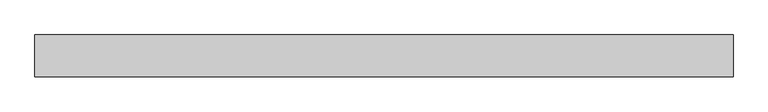
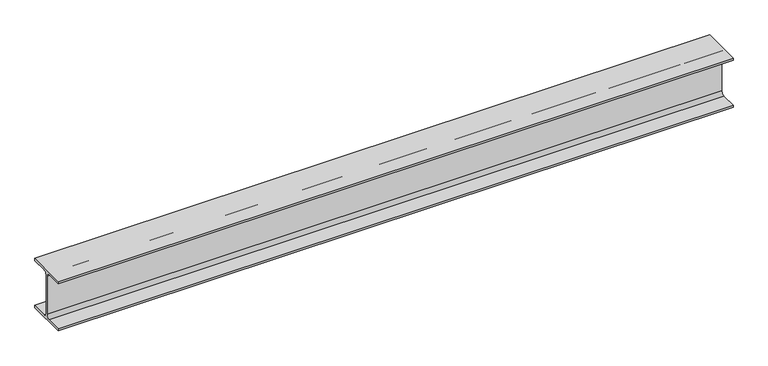
"""IFC4 building model written with IfcOpenShell, lengths in millimetres: beam geometry, 0912_Steel Framing_H-KSD3502 : H_SB_ASB_H-194x150x6x9."""

import ifcopenshell
import ifcopenshell.guid

model = None  # the IFC model being written
_history = None  # IfcOwnerHistory: only IFC2X3 demands one
_inside = {}  # id of a spatial element -> (the spatial element, [elements in it])
_under = {}  # id of a project, library or spatial element -> (it, [spatial elements below it])
_declared = {}  # id of a project -> (the project, [libraries it declares])
_typed = {}  # id of a type object -> (the type object, [elements of that type])
_made_of = {}  # id of a material, layer set ... -> (it, [elements and type objects made of it])


def new_model(schema):
    """Start an empty IFC model of exactly this schema.

    Asked for "IFC4X3", IfcOpenShell would pick the latest addendum, in which some entities
    have other attributes; the version numbers below select the first issue.
    IFC2X3 requires an IfcOwnerHistory on every rooted entity: one is made here for all.
    """
    global model, _history
    if schema == "IFC4X3":
        model = ifcopenshell.file(schema_version=(4, 3, 0, 0))
    else:
        model = ifcopenshell.file(schema=schema)
    _inside.clear()
    _under.clear()
    _declared.clear()
    _typed.clear()
    _made_of.clear()
    _history = None
    if model.schema == "IFC2X3":
        org = make("IfcOrganization", Name="unknown")
        user = make(
            "IfcPersonAndOrganization",
            ThePerson=make("IfcPerson", FamilyName="unknown"),
            TheOrganization=org,
        )
        app = make(
            "IfcApplication",
            ApplicationDeveloper=org,
            Version="unknown",
            ApplicationFullName="unknown",
            ApplicationIdentifier="unknown",
        )
        _history = make(
            "IfcOwnerHistory",
            OwningUser=user,
            OwningApplication=app,
            ChangeAction="ADDED",
            CreationDate=0,
        )
    return model


def make(cls, **values):
    """One entity of the class cls with the attributes given. An attribute that is None is left unset."""
    return model.create_entity(
        cls, **{name: value for name, value in values.items() if value is not None}
    )


def rooted(cls, **values):
    """An entity with a GlobalId (a new one), such as an element, a storey or a relation."""
    return make(cls, GlobalId=ifcopenshell.guid.new(), OwnerHistory=_history, **values)


def si_unit(unit_type, name, prefix=None):
    """IfcSIUnit, for example si_unit("LENGTHUNIT", "METRE", prefix="MILLI")."""
    return make("IfcSIUnit", UnitType=unit_type, Prefix=prefix, Name=name)


def assignment(units):
    """IfcUnitAssignment: the units of a project."""
    return None if units is None else make("IfcUnitAssignment", Units=units)


def point(xyz):
    """IfcCartesianPoint."""
    return None if xyz is None else make("IfcCartesianPoint", Coordinates=xyz)


def direction(xyz):
    """IfcDirection."""
    return None if xyz is None else make("IfcDirection", DirectionRatios=xyz)


def frame(location, z_axis=None, x_axis=None):
    """IfcAxis2Placement3D, a coordinate frame: its origin and axes. An axis left out is left unset."""
    return make(
        "IfcAxis2Placement3D",
        Location=point(location),
        Axis=direction(z_axis),
        RefDirection=direction(x_axis),
    )


def frame_2d(location, x_axis=None):
    """IfcAxis2Placement2D, a coordinate frame in the plane: its origin and x axis."""
    return make(
        "IfcAxis2Placement2D", Location=point(location), RefDirection=direction(x_axis)
    )


def origin():
    """The frame at (0, 0, 0) with its axes left unset."""
    return frame((0.0, 0.0, 0.0))


def place(relative_to, where):
    """IfcLocalPlacement: puts the frame where relative to a parent placement (None: the world)."""
    return make(
        "IfcLocalPlacement", PlacementRelTo=relative_to, RelativePlacement=where
    )


def context(
    kind, dimensions, precision=None, world=None, true_north=None, identifier=None
):
    """IfcGeometricRepresentationContext, for example the 3D "Model" context."""
    return make(
        "IfcGeometricRepresentationContext",
        ContextIdentifier=identifier,
        ContextType=kind,
        CoordinateSpaceDimension=dimensions,
        Precision=precision,
        WorldCoordinateSystem=world,
        TrueNorth=true_north,
    )


def project(units=None, contexts=None):
    """IfcProject with its units and contexts."""
    return rooted(
        "IfcProject",
        Name="project",
        RepresentationContexts=contexts,
        UnitsInContext=assignment(units),
    )


def spatial(cls, under=None, at=None, **own):
    """A site, building, storey or space (cls), placed at a placement, below another one or the project."""
    s = rooted(cls, ObjectPlacement=at, **own)
    if under is not None:
        _under.setdefault(under.id(), (under, []))[1].append(s)
    return s


def polyline(points):
    """IfcPolyline through the points."""
    return make("IfcPolyline", Points=[point(p) for p in points])


def circle_curve(where, radius):
    """IfcCircle in the frame where."""
    return make("IfcCircle", Position=where, Radius=radius)


def trimmed(basis, trim1, trim2, sense, master):
    """IfcTrimmedCurve: the piece of a basis curve between two trims."""
    return make(
        "IfcTrimmedCurve",
        BasisCurve=basis,
        Trim1=trim1,
        Trim2=trim2,
        SenseAgreement=sense,
        MasterRepresentation=master,
    )


def segment(curve, same_sense, transition):
    """IfcCompositeCurveSegment."""
    return make(
        "IfcCompositeCurveSegment",
        Transition=transition,
        SameSense=same_sense,
        ParentCurve=curve,
    )


def composite_curve(segments, self_intersect=None):
    """IfcCompositeCurve: segments joined end to end."""
    return make("IfcCompositeCurve", Segments=segments, SelfIntersect=self_intersect)


def outline(outer, holes=None, kind="AREA"):
    """IfcArbitraryClosedProfileDef: a profile drawn as a closed curve; with holes, ...WithVoids."""
    if holes is None:
        return make("IfcArbitraryClosedProfileDef", ProfileType=kind, OuterCurve=outer)
    return make(
        "IfcArbitraryProfileDefWithVoids",
        ProfileType=kind,
        OuterCurve=outer,
        InnerCurves=holes,
    )


def extrude(swept, where, along, depth):
    """IfcExtrudedAreaSolid: the profile swept, set in the frame where, extruded along a direction by depth."""
    return make(
        "IfcExtrudedAreaSolid",
        SweptArea=swept,
        Position=where,
        ExtrudedDirection=direction(along),
        Depth=depth,
    )


def shape(context_of_items, identifier, shape_type, items):
    """IfcShapeRepresentation: the items that make up one representation, for example the "Body"."""
    return make(
        "IfcShapeRepresentation",
        ContextOfItems=context_of_items,
        RepresentationIdentifier=identifier,
        RepresentationType=shape_type,
        Items=items,
    )


def source(mapping_origin, context_of_items, identifier, shape_type, items):
    """IfcRepresentationMap: a shape defined once, which mapped items show again and again."""
    return make(
        "IfcRepresentationMap",
        MappingOrigin=mapping_origin,
        MappedRepresentation=shape(context_of_items, identifier, shape_type, items),
    )


def transform(
    local_origin,
    x_axis=None,
    y_axis=None,
    z_axis=None,
    scale=None,
    scale2=None,
    scale3=None,
    uniform=True,
):
    """IfcCartesianTransformationOperator3D, or its non-uniform kind. x_axis, y_axis, z_axis: its Axis1, 2, 3."""
    if uniform:
        return make(
            "IfcCartesianTransformationOperator3D",
            Axis1=direction(x_axis),
            Axis2=direction(y_axis),
            LocalOrigin=point(local_origin),
            Scale=scale,
            Axis3=direction(z_axis),
        )
    return make(
        "IfcCartesianTransformationOperator3DnonUniform",
        Axis1=direction(x_axis),
        Axis2=direction(y_axis),
        LocalOrigin=point(local_origin),
        Scale=scale,
        Axis3=direction(z_axis),
        Scale2=scale2,
        Scale3=scale3,
    )


def mapped(mapping_source, mapping_target):
    """IfcMappedItem: shows the shape of a source again, moved by a transform."""
    return make(
        "IfcMappedItem", MappingSource=mapping_source, MappingTarget=mapping_target
    )


def made_of(thing, what):
    """Note that an element or type object is made of a material, layer set ...; save() writes the relation."""
    if what is not None:
        _made_of.setdefault(what.id(), (what, []))[1].append(thing)
    return thing


def element(
    cls,
    number,
    at=None,
    inside=None,
    cuts=None,
    type_object=None,
    material=None,
    context=None,
    identifier="Body",
    shape_type=None,
    held_by="IfcProductDefinitionShape",
    body=None,
    shapes=None,
    **own,
):
    """One element of the class cls, such as IfcWall. Its Tag is "e" and its number.

    at: its placement. inside: the storey or other place that contains it. cuts: it is an
    opening in that element (IfcRelVoidsElement). A single representation is given by context,
    identifier, shape_type and body (its items); several are given by shapes. held_by: the class
    of the entity that holds the representations. save() writes the other relations.
    """
    e = rooted(cls, Tag="e%d" % number, ObjectPlacement=at, **own)
    if body is not None:
        shapes = [shape(context, identifier, shape_type, body)]
    if shapes is not None:
        e.Representation = make(held_by, Representations=shapes)
    if inside is not None:
        _inside.setdefault(inside.id(), (inside, []))[1].append(e)
    if cuts is not None:
        rooted(
            "IfcRelVoidsElement", RelatingBuildingElement=cuts, RelatedOpeningElement=e
        )
    if type_object is not None:
        _typed.setdefault(type_object.id(), (type_object, []))[1].append(e)
    return made_of(e, material)


def aggregate(whole, parts):
    """IfcRelAggregates: a whole, such as a stair, and the parts it consists of."""
    return rooted("IfcRelAggregates", RelatingObject=whole, RelatedObjects=parts)


def save(model, path):
    """Write the relations noted so far, then the file.

    IfcRelAggregates (storeys below a building ...), IfcRelContainedInSpatialStructure (elements
    in a storey), IfcRelDefinesByType, IfcRelAssociatesMaterial and IfcRelDeclares: one each for
    every whole, place, type object, material and project.
    """
    for whole, parts in _under.values():
        aggregate(whole, parts)
    for where, things in _inside.values():
        rooted(
            "IfcRelContainedInSpatialStructure",
            RelatedElements=things,
            RelatingStructure=where,
        )
    for kind, things in _typed.values():
        rooted("IfcRelDefinesByType", RelatedObjects=things, RelatingType=kind)
    for what, things in _made_of.values():
        rooted("IfcRelAssociatesMaterial", RelatedObjects=things, RelatingMaterial=what)
    for by, libraries in _declared.values():
        rooted("IfcRelDeclares", RelatingContext=by, RelatedDefinitions=libraries)
    model.write(path)


def beam_2ed9de13(model_context):
    return source(origin(), model_context, "Body", "SweptSolid", [
        extrude(outline(composite_curve([segment(polyline([(-75.0, -88.0), (-16.0, -88.0)]), True, "CONTINUOUS"), segment(trimmed(circle_curve(frame_2d((-16.0, -75.0)), 13.0), [point((-16.0, -88.0))], [point((-3.0, -75.0))], True, "CARTESIAN"), True, "CONTINUOUS"), segment(polyline([(-3.0, -75.0), (-3.0, 75.0)]), True, "CONTINUOUS"), segment(trimmed(circle_curve(frame_2d((-16.0, 75.0)), 13.0), [point((-3.0, 75.0))], [point((-16.0, 88.0))], True, "CARTESIAN"), True, "CONTINUOUS"), segment(polyline([(-16.0, 88.0), (-75.0, 88.0), (-75.0, 97.0), (75.0, 97.0), (75.0, 88.0), (16.0, 88.0)]), True, "CONTINUOUS"), segment(trimmed(circle_curve(frame_2d((16.0, 75.0)), 13.0), [point((16.0, 88.0))], [point((3.0, 75.0))], True, "CARTESIAN"), True, "CONTINUOUS"), segment(polyline([(3.0, 75.0), (3.0, -75.0)]), True, "CONTINUOUS"), segment(trimmed(circle_curve(frame_2d((16.0, -75.0)), 13.0), [point((3.0, -75.0))], [point((16.0, -88.0))], True, "CARTESIAN"), True, "CONTINUOUS"), segment(polyline([(16.0, -88.0), (75.0, -88.0), (75.0, -97.0), (-75.0, -97.0), (-75.0, -88.0)]), True, "CONTINUOUS")], self_intersect=False)), frame((-1253.7727018, 0.0, 0.0), z_axis=(1.0, 0.0, 0.0), x_axis=(0.0, 1.0, 0.0)), (0.0, 0.0, 1.0), 2507.5454037),
    ])


if __name__ == "__main__":
    model = new_model("IFC4")
    model_context = context("Model", 3, world=origin())
    ifc_project = project(units=[si_unit("LENGTHUNIT", "METRE", prefix="MILLI")], contexts=[model_context])
    site = spatial("IfcSite", under=ifc_project)
    building = spatial("IfcBuilding", under=site)
    placement = place(None, origin())
    beam_shape = beam_2ed9de13(model_context)
    element("IfcBeam", 1, ObjectType="0912_Steel Framing_H-KSD3502 : H_SB_ASB_H-194x150x6x9", at=placement, inside=building, context=model_context, shape_type="MappedRepresentation", body=[
        mapped(beam_shape, transform((0.0, 0.0, 0.0), x_axis=(1.0, 0.0, 0.0), y_axis=(0.0, 1.0, 0.0), z_axis=(0.0, 0.0, 1.0))),
    ])
    save(model, "model.ifc")

# Revit data of these elements
# Type "0912_Steel Framing_H-KSD3502 : H_SB_ASB_H-194x150x6x9"
#   H_WM Code_1 = "S01AA002-00001 | Main Steel Structure Fabrication Work | Shelter/Building | Medium Steel - Standard (90KG/M>Weight≥30KG/M) | Material: (   )"
#   H_WM Code_2 = "S03AA028-00001 | Main Steel Structure Erection Work | Shelter/Building | Medium Steel (90KG/M>Weight≥30KG/M) | Material: (   )"
#   H_WM Code_3 = "S01AA010-00001 | Main Steel Structure Fabrication Work | Shelter/Building | Steel Painting/Coating | for Non-Fireproofed Steel Surface, Surface Preparation, Primer, Second & Final Coat | Material: (   )"
#   H_Q'ty Cal Type Tag = "SB-Q2"
#   Width = 15.0 cm
#   Web Thickness = 0.6 cm
#   Web Fillet = 1.3 cm
#   Warping Constant = 43316.0 cm⁶
#   W = 0
#   Torsional Moment of Inertia = 8.622 cm⁴
#   Section Area = 39.01 cm²
#   Plastic Modulus weak axis = 104.0 cm³
#   Plastic Modulus strong axis = 309.0 cm³
#   Perimeter = 0.95 m²/m
#   Nominal Weight = 30.60 kgf/m
#   Moment of Inertia weak axis = 507.00 cm⁴
#   Moment of Inertia strong axis = 2690.00 cm⁴
#   Height = 19.4 cm
#   Flange Thickness = 0.9 cm
#   Elastic Modulus weak axis = 67.6 cm³
#   Elastic Modulus strong axis = 277.0 cm³
#   Centroid Vertical = 9.7 cm
#   Centroid Horizontal = 7.5 cm
#   Ix = 26900000
#   Length [instance default] = 1.5240 m
#   Zx = 309000
#   b = 0.1500 m
#   h = 0.1940 m
#   r = 0.0130 m
#   s = 0.0060 m
#   t = 0.0090 m
#   A = 0.003901 m²
#   Structural Material [instance default] = Steel, 45-345
#   Assembly Code = ""
# Element 1 (IfcBeam, "0912_Steel Framing_H-KSD3502 : H_SB_ASB_H-194x150x6x9")
#   Structural Material = none
# Materials
#   "Steel, 45-345": class "Metal", colour RGB 189 187 185, transparency 0, Description = "Steel 345 MPa", Cost = 0
